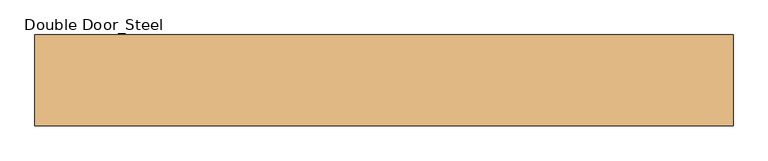
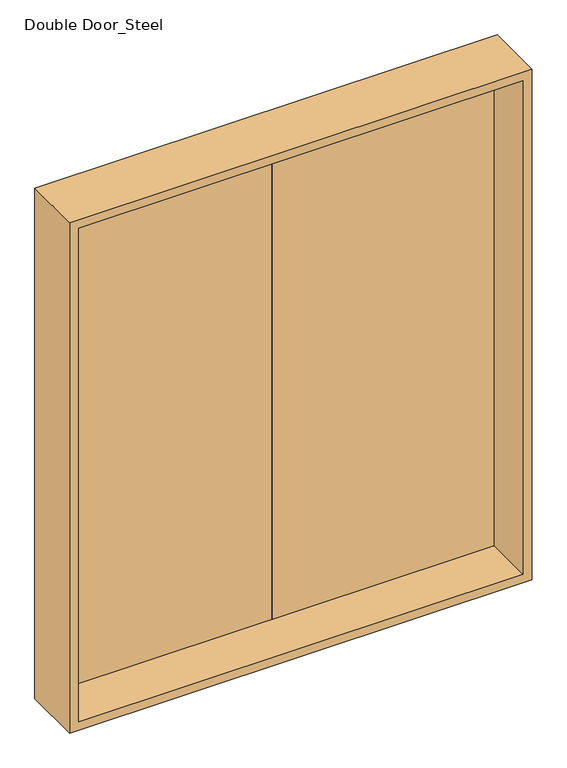
"""IFC4 building model written with IfcOpenShell, lengths in millimetres: door geometry, Double Door_Steel : H_DR_AR_B12_Double Door_Steel_W2000xH2100."""

from ifc_helpers import new_model, si_unit, frame, origin, place, context, project, spatial, polyline, outline, extrude, faceted_brep, source, transform, mapped, element, save


def double_door_steel_ece7098f(model_context):
    return source(origin(), model_context, "Body", "SolidModel", [
        extrude(outline(polyline([(880.0, 77.0), (0.0, 77.0), (0.0, 117.0), (880.0, 117.0), (880.0, 77.0)])), frame((0.0, 0.0, 20.0), z_axis=(0.0, 0.0, 1.0), x_axis=(1.0, 0.0, 0.0)), (0.0, 0.0, 1.0), 2060.0),
        extrude(outline(polyline([(0.0, 77.0), (-880.0, 77.0), (-880.0, 117.0), (0.0, 117.0), (0.0, 77.0)])), frame((0.0, 0.0, 20.0), z_axis=(0.0, 0.0, 1.0), x_axis=(1.0, 0.0, 0.0)), (0.0, 0.0, 1.0), 2060.0),
        faceted_brep([(900.0, -117.0, 2100.0), (900.0, 117.0, 2100.0), (-900.0, 117.0, 2100.0), (-900.0, -117.0, 2100.0), (865.0, 77.0, 2065.0), (865.0, -117.0, 2065.0), (-865.0, -117.0, 2065.0), (-865.0, 77.0, 2065.0), (880.0, 117.0, 2080.0), (880.0, 77.0, 2080.0), (-880.0, 77.0, 2080.0), (-880.0, 117.0, 2080.0), (-900.0, 117.0, 0.0), (-900.0, -117.0, 0.0), (-865.0, -117.0, 35.0), (-865.0, 77.0, 35.0), (-880.0, 77.0, 20.0), (-880.0, 117.0, 20.0), (900.0, 117.0, 0.0), (880.0, 117.0, 20.0), (900.0, -117.0, 0.0), (865.0, -117.0, 35.0), (865.0, 77.0, 35.0), (880.0, 77.0, 20.0)], [[[0, 1, 2, 3]], [[4, 5, 6, 7]], [[8, 9, 10, 11]], [[3, 2, 12, 13]], [[7, 6, 14, 15]], [[11, 10, 16, 17]], [[18, 12, 2, 1], [8, 11, 17, 19]], [[13, 12, 18, 20]], [[0, 3, 13, 20], [21, 14, 6, 5]], [[15, 14, 21, 22]], [[23, 16, 10, 9], [4, 7, 15, 22]], [[17, 16, 23, 19]], [[20, 18, 1, 0]], [[22, 21, 5, 4]], [[19, 23, 9, 8]]]),
    ])


if __name__ == "__main__":
    model = new_model("IFC4")
    model_context = context("Model", 3, world=origin())
    ifc_project = project(units=[si_unit("LENGTHUNIT", "METRE", prefix="MILLI")], contexts=[model_context])
    site = spatial("IfcSite", under=ifc_project)
    building = spatial("IfcBuilding", under=site)
    placement = place(None, origin())
    double_door_steel_shape = double_door_steel_ece7098f(model_context)
    element("IfcDoor", 1, ObjectType="Double Door_Steel : H_DR_AR_B12_Double Door_Steel_W2000xH2100", at=placement, inside=building, context=model_context, shape_type="MappedRepresentation", body=[
        mapped(double_door_steel_shape, transform((0.0, 0.0, 0.0), x_axis=(1.0, 0.0, 0.0), y_axis=(0.0, 1.0, 0.0), z_axis=(0.0, 0.0, 1.0))),
    ])
    save(model, "model.ifc")

# Revit data of these elements
# Type "Double Door_Steel : H_DR_AR_B12_Double Door_Steel_W2000xH2100"
#   Type Mark = ""
#   프레임 = ""
#   철물 = ""
#   유리/마감 = ""
#   위치/개소 = ""
#   부호 = "1/SD"
#   문번호 = ""
#   문기호 = "SD"
#   Analytic Construction = "<None>"
#   Height = 2100 mm
#   Width = 1800 mm
#   Define Thermal Properties by = 1
#   문 틀 = none
#   문 = none
#   Function = (empty or 0)
#   Assembly Code = ""
#   Wall Closure = (empty or 0)
